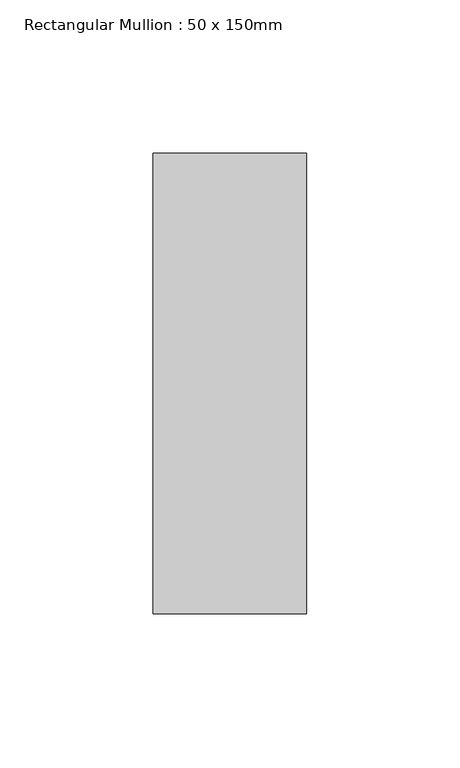
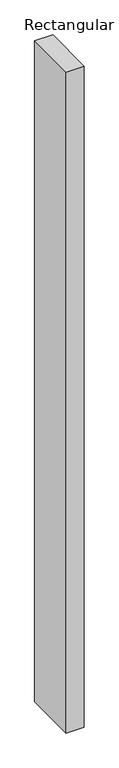
"""IFC4 building model written with IfcOpenShell, lengths in millimetres: member geometry, Rectangular Mullion : 50 x 150mm."""

from ifc_helpers import new_model, si_unit, frame, origin, place, context, project, spatial, polyline, outline, extrude, source, transform, mapped, element, save


def rectangular_mullion_50_x_150mm_3bfcaf8b(model_context):
    return source(origin(), model_context, "Body", "SweptSolid", [
        extrude(outline(polyline([(25.0, 75.0), (25.0, -75.0), (-25.0, -75.0), (-25.0, 75.0), (25.0, 75.0)])), frame((0.0, 0.0, -1925.0000003), z_axis=(0.0, 0.0, 1.0), x_axis=(1.0, 0.0, 0.0)), (0.0, 0.0, 1.0), 1925.0000003),
    ])


if __name__ == "__main__":
    model = new_model("IFC4")
    model_context = context("Model", 3, world=origin())
    ifc_project = project(units=[si_unit("LENGTHUNIT", "METRE", prefix="MILLI")], contexts=[model_context])
    site = spatial("IfcSite", under=ifc_project)
    building = spatial("IfcBuilding", under=site)
    placement = place(None, origin())
    rectangular_mullion_50_x_150mm_shape = rectangular_mullion_50_x_150mm_3bfcaf8b(model_context)
    element("IfcMember", 1, ObjectType="Rectangular Mullion : 50 x 150mm", at=placement, inside=building, context=model_context, shape_type="MappedRepresentation", body=[
        mapped(rectangular_mullion_50_x_150mm_shape, transform((0.0, 0.0, 0.0), x_axis=(1.0, 0.0, 0.0), y_axis=(0.0, 1.0, 0.0), z_axis=(0.0, 0.0, 1.0))),
    ])
    save(model, "model.ifc")

# Revit data of these elements
# Type "Rectangular Mullion : 50 x 150mm"
#   built-in parameter 1007304 = 0.492126 (stored number, unit not read)
#   built-in parameter 1007301 = 0.082021 (stored number, unit not read)
#   built-in parameter 1007300 = 0.082021 (stored number, unit not read)
# Element 1 (IfcMember, "Rectangular Mullion : 50 x 150mm")
#   Materials on its faces: "Metal - Aluminium"
# Materials
#   "Metal - Aluminium": class "Metal", colour RGB 247 247 247, transparency 0
